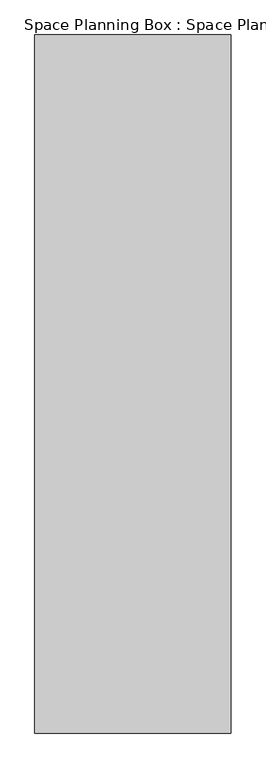
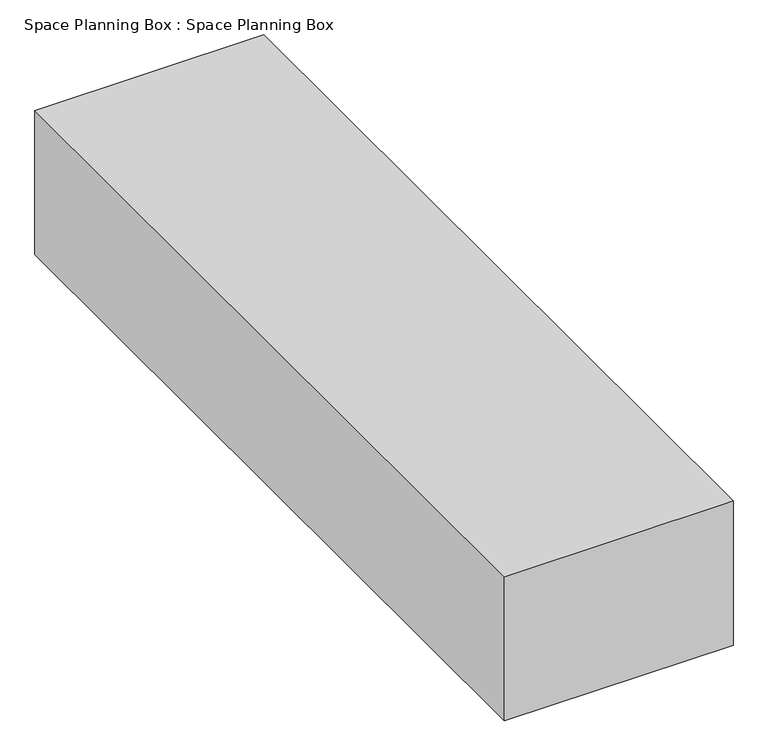
"""IFC4 building model written with IfcOpenShell, lengths in millimetres: proxy geometry, Space Planning Box : Space Planning Box."""

from ifc_helpers import new_model, si_unit, origin, origin_with_axes, place, context, project, spatial, polyline, outline, extrude, source, transform, mapped, element, save


def space_planning_box_space_planning_box_57c7875f(model_context):
    return source(origin(), model_context, "Body", "SweptSolid", [
        extrude(outline(polyline([(4500.0, 16000.0), (4500.0, -16000.0), (-4500.0, -16000.0), (-4500.0, 16000.0), (4500.0, 16000.0)])), origin_with_axes(), (0.0, 0.0, 1.0), 6000.0),
    ])


if __name__ == "__main__":
    model = new_model("IFC4")
    model_context = context("Model", 3, world=origin())
    ifc_project = project(units=[si_unit("LENGTHUNIT", "METRE", prefix="MILLI")], contexts=[model_context])
    site = spatial("IfcSite", under=ifc_project)
    building = spatial("IfcBuilding", under=site)
    placement = place(None, origin())
    space_planning_box_space_planning_box_shape = space_planning_box_space_planning_box_57c7875f(model_context)
    element("IfcBuildingElementProxy", 1, Name="Space Planning Box : Space Planning Box", ObjectType="Space Planning Box : Space Planning Box", at=placement, inside=building, context=model_context, shape_type="MappedRepresentation", body=[
        mapped(space_planning_box_space_planning_box_shape, transform((0.0, 0.0, 0.0), x_axis=(1.0, 0.0, 0.0), y_axis=(0.0, 1.0, 0.0), z_axis=(0.0, 0.0, 1.0))),
    ])
    save(model, "model.ifc")

# Revit data of these elements
# Type "Space Planning Box : Space Planning Box"
#   Type Comments = "..."
#   Room Name [instance default] = "?"
#   Assembly Code = "..."
#   Width [instance default] = 1524 mm
#   Program Area [instance default] = 0 m²
#   Length [instance default] = 1524 mm
#   Height [instance default] = 1524 mm
#   Area [instance default] = 2.32258 m²
#   Fill Color [instance default] = Cyan
#   Default Elevation = 0
# Element 1 (IfcBuildingElementProxy, "Space Planning Box : Space Planning Box")
#   Room Name = "Central Control Room"
#   Width = 9000 mm
#   Program Area = 288 m²
#   Length = 32000 mm
#   Height = 6000 mm
#   Area = 288 m²
#   Fill Color = Lime
#   Materials on its faces: "Lime"
# Materials
#   "Cyan": class "Generic", colour RGB 0 255 255, transparency 0.2, Cost = 0
#   "Lime": class "Generic", colour RGB 0 255 0, transparency 0.2, Cost = 0
